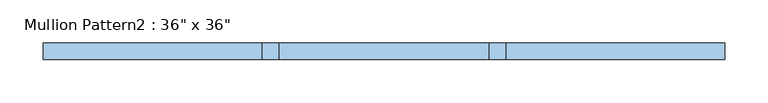
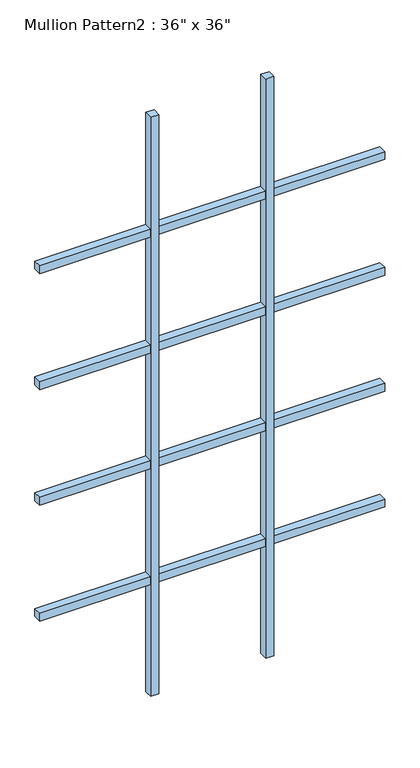
"""IFC4 building model written with IfcOpenShell, lengths in millimetres: window geometry."""

from ifc_helpers import new_model, si_unit, frame, origin, place, context, project, spatial, polyline, outline, extrude, source, transform, mapped, element, save


def window_f4a03a44(model_context):
    return source(origin(), model_context, "Body", "SweptSolid", [
        extrude(outline(polyline([(140.7583333, -19.05), (121.7083333, -19.05), (121.7083333, 0.0), (140.7583333, 0.0), (140.7583333, -19.05)])), frame((0.0, 0.0, 762.0), z_axis=(0.0, 0.0, 1.0), x_axis=(1.0, 0.0, 0.0)), (0.0, 0.0, 1.0), 1397.0),
        extrude(outline(polyline([(-121.7083333, -19.05), (-140.7583333, -19.05), (-140.7583333, 0.0), (-121.7083333, 0.0), (-121.7083333, -19.05)])), frame((0.0, 0.0, 762.0), z_axis=(0.0, 0.0, 1.0), x_axis=(1.0, 0.0, 0.0)), (0.0, 0.0, 1.0), 1397.0),
        extrude(outline(polyline([(393.7, -19.05), (-393.7, -19.05), (-393.7, 0.0), (393.7, 0.0), (393.7, -19.05)])), frame((0.0, 0.0, 1590.675), z_axis=(0.0, 0.0, 1.0), x_axis=(1.0, 0.0, 0.0)), (0.0, 0.0, 1.0), 19.05),
        extrude(outline(polyline([(393.7, -19.05), (-393.7, -19.05), (-393.7, 0.0), (393.7, 0.0), (393.7, -19.05)])), frame((0.0, 0.0, 1311.275), z_axis=(0.0, 0.0, 1.0), x_axis=(1.0, 0.0, 0.0)), (0.0, 0.0, 1.0), 19.05),
        extrude(outline(polyline([(393.7, -19.05), (-393.7, -19.05), (-393.7, 0.0), (393.7, 0.0), (393.7, -19.05)])), frame((0.0, 0.0, 1870.075), z_axis=(0.0, 0.0, 1.0), x_axis=(1.0, 0.0, 0.0)), (0.0, 0.0, 1.0), 19.05),
        extrude(outline(polyline([(393.7, -19.05), (-393.7, -19.05), (-393.7, 0.0), (393.7, 0.0), (393.7, -19.05)])), frame((0.0, 0.0, 1031.875), z_axis=(0.0, 0.0, 1.0), x_axis=(1.0, 0.0, 0.0)), (0.0, 0.0, 1.0), 19.05),
    ])


if __name__ == "__main__":
    model = new_model("IFC4")
    model_context = context("Model", 3, world=origin())
    ifc_project = project(units=[si_unit("LENGTHUNIT", "METRE", prefix="MILLI")], contexts=[model_context])
    site = spatial("IfcSite", under=ifc_project)
    building = spatial("IfcBuilding", under=site)
    placement = place(None, origin())
    window_shape = window_f4a03a44(model_context)
    element("IfcWindow", 1, ObjectType="Mullion Pattern2 : 36\" x 36\"", at=placement, inside=building, context=model_context, shape_type="MappedRepresentation", body=[
        mapped(window_shape, transform((0.0, 0.0, 0.0), x_axis=(1.0, 0.0, 0.0), y_axis=(0.0, 1.0, 0.0), z_axis=(0.0, 0.0, 1.0))),
    ])
    save(model, "model.ifc")

# Revit data of these elements
# Type "Mullion Pattern2 : 36\" x 36\""
#   Type Mark = "30"
#   Analytic Construction = "<None>"
#   Width = 2.583333 ft
#   Height = 4.583333 ft
#   Vertical Lites = 5
#   Mullion Single Visiblity - Horz = no
#   Mullion Single Visibilty - Vert = no
#   Mullion Multi Visibility - Horz = yes
#   Mullion Multi Visibility - Vert = yes
#   Horizontal Lites = 3
#   Mullion Material = Sash
# Element 1 (IfcWindow, "Mullion Pattern2 : 36\" x 36\"")
#   Materials on its faces: "Sash"
# Materials
#   "Sash": class "Wood", colour RGB 224 178 126, transparency 0, Cost = 0
